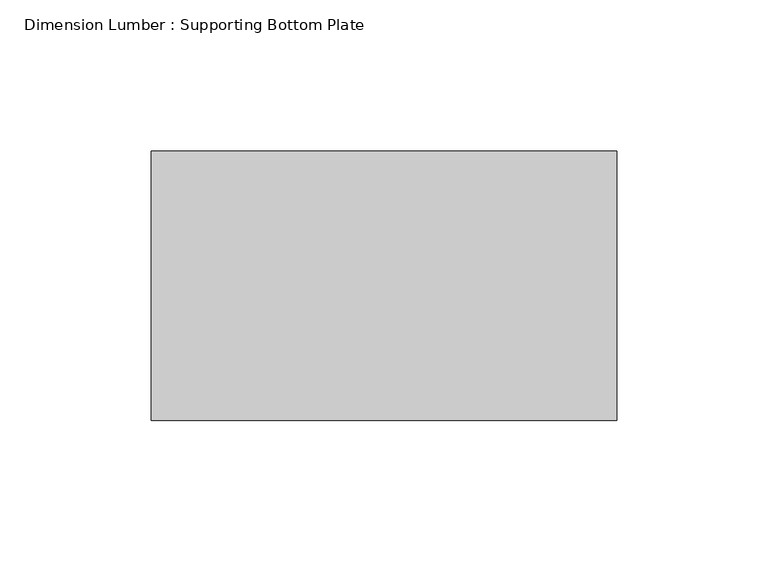
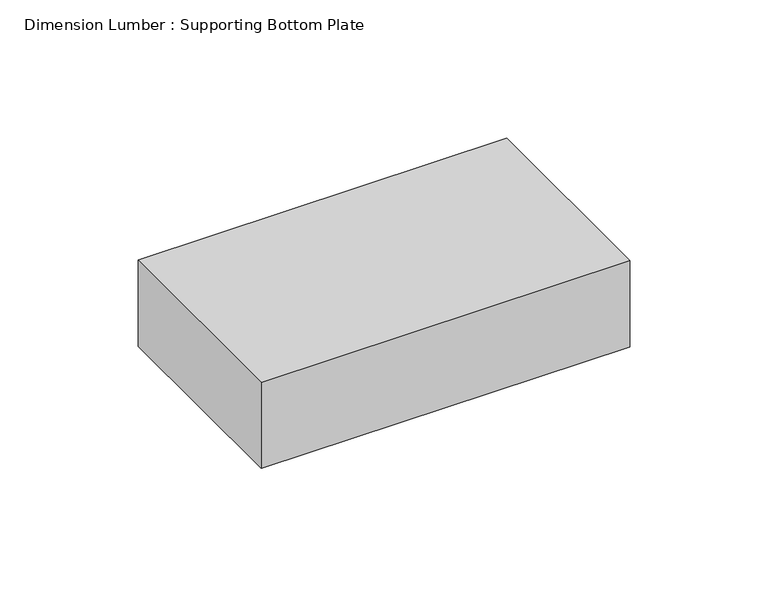
"""IFC4 building model written with IfcOpenShell, lengths in millimetres: beam geometry, Dimension Lumber : Supporting Bottom Plate."""

from ifc_helpers import new_model, si_unit, frame, origin, place, context, project, spatial, polyline, outline, extrude, source, transform, mapped, element, save


def dimension_lumber_supporting_bottom_plate_937476ce(model_context):
    return source(origin(), model_context, "Body", "SweptSolid", [
        extrude(outline(polyline([(53.975, 44.45), (53.975, -44.45), (-99.615625, -44.45), (-99.615625, 44.45), (53.975, 44.45)])), frame((0.0, 0.0, -19.05), z_axis=(0.0, 0.0, 1.0), x_axis=(1.0, 0.0, 0.0)), (0.0, 0.0, 1.0), 38.1),
    ])


if __name__ == "__main__":
    model = new_model("IFC4")
    model_context = context("Model", 3, world=origin())
    ifc_project = project(units=[si_unit("LENGTHUNIT", "METRE", prefix="MILLI")], contexts=[model_context])
    site = spatial("IfcSite", under=ifc_project)
    building = spatial("IfcBuilding", under=site)
    placement = place(None, origin())
    dimension_lumber_supporting_bottom_plate_shape = dimension_lumber_supporting_bottom_plate_937476ce(model_context)
    element("IfcBeam", 1, ObjectType="Dimension Lumber : Supporting Bottom Plate", at=placement, inside=building, context=model_context, shape_type="MappedRepresentation", body=[
        mapped(dimension_lumber_supporting_bottom_plate_shape, transform((0.0, 0.0, 0.0), x_axis=(1.0, 0.0, 0.0), y_axis=(0.0, 1.0, 0.0), z_axis=(0.0, 0.0, 1.0))),
    ])
    save(model, "model.ifc")

# Revit data of these elements
# Type "Dimension Lumber : Supporting Bottom Plate"
#   Assembly Code = "B10"
#   A = 0.0364583 SF
#   Length [instance default] = 5' - 0"
#   b = 0' - 3 1/2"
#   d = 0' - 1 1/2"
#   Structural Material [instance default] = Softwood, Lumber
# Element 1 (IfcBeam, "Dimension Lumber : Supporting Bottom Plate")
#   Structural Material = Douglas Fir #2
#   Materials on its faces: "Douglas Fir #2"
# Materials
#   "Softwood, Lumber": class "Wood", colour RGB 223 192 134, transparency 0, Description = "Pinus Echinata", Cost = 0
#   "Douglas Fir #2": class "Wood", colour RGB 223 192 134, transparency 0, Description = "Pinus Echinata", Cost = 0
